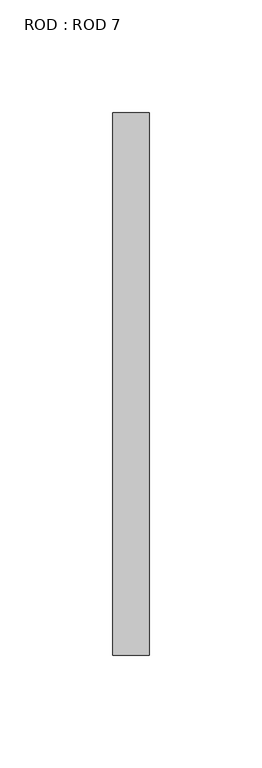
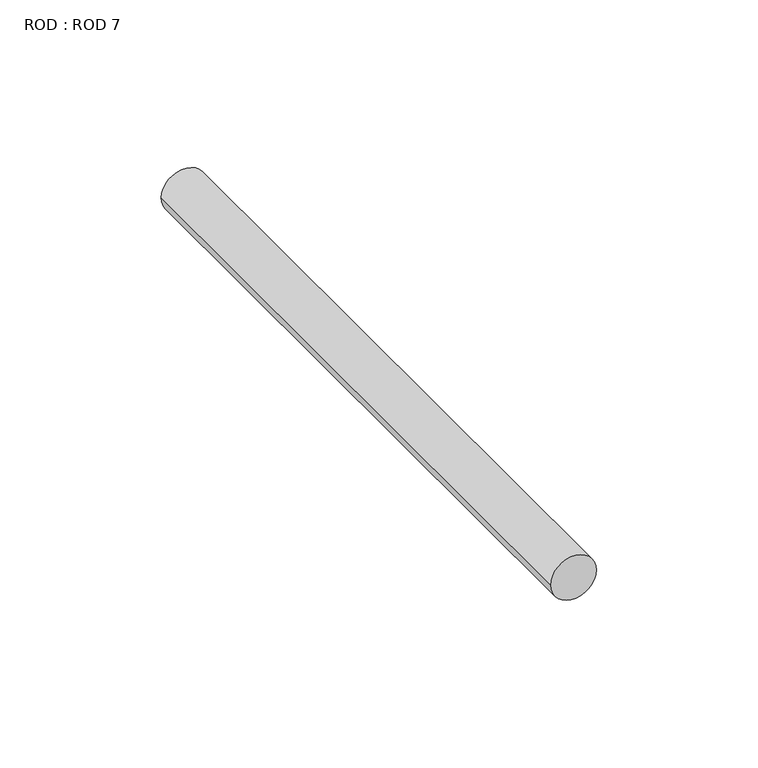
"""IFC4 building model written with IfcOpenShell, lengths in millimetres: proxy geometry, ROD : ROD 7."""

from ifc_helpers import new_model, si_unit, point, frame, origin, origin_2d, place, context, project, spatial, circle_curve, trimmed, segment, composite_curve, outline, extrude, source, transform, mapped, element, save


def rod_rod_7_7008c9f0(model_context):
    return source(origin(), model_context, "Body", "SweptSolid", [
        extrude(outline(composite_curve([segment(trimmed(circle_curve(origin_2d(), 8.1359375), [point((0.0, 8.1359375))], [point((0.0, -8.1359375))], False, "CARTESIAN"), True, "CONTINUOUS"), segment(trimmed(circle_curve(origin_2d(), 8.1359375), [point((0.0, -8.1359375))], [point((0.0, 8.1359375))], False, "CARTESIAN"), True, "CONTINUOUS")], self_intersect=False)), frame((0.0, -152.4, 0.0), z_axis=(0.0, 1.0, 0.0), x_axis=(0.0, 0.0, 1.0)), (0.0, 0.0, 1.0), 241.3),
    ])


if __name__ == "__main__":
    model = new_model("IFC4")
    model_context = context("Model", 3, world=origin())
    ifc_project = project(units=[si_unit("LENGTHUNIT", "METRE", prefix="MILLI")], contexts=[model_context])
    site = spatial("IfcSite", under=ifc_project)
    building = spatial("IfcBuilding", under=site)
    placement = place(None, origin())
    rod_rod_7_shape = rod_rod_7_7008c9f0(model_context)
    element("IfcBuildingElementProxy", 1, Name="ROD : ROD 7", ObjectType="ROD : ROD 7", at=placement, inside=building, context=model_context, shape_type="MappedRepresentation", body=[
        mapped(rod_rod_7_shape, transform((0.0, 0.0, 0.0), x_axis=(1.0, 0.0, 0.0), y_axis=(0.0, 1.0, 0.0), z_axis=(0.0, 0.0, 1.0))),
    ])
    save(model, "model.ifc")

# Revit data of these elements
# Type "ROD : ROD 7"
#   lenght = 0' - 9 1/2"
#   Radius = 0' - 0 41/128"
#   material [instance default] = 3/4" GALV. THRU BOLTS
# Materials
#   "3/4\" GALV. THRU BOLTS": class "Generic", colour RGB 105 69 171, transparency 0, Cost = 0
